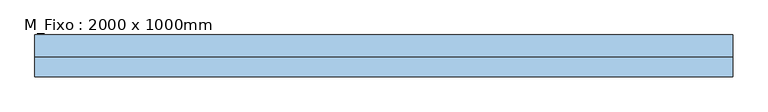
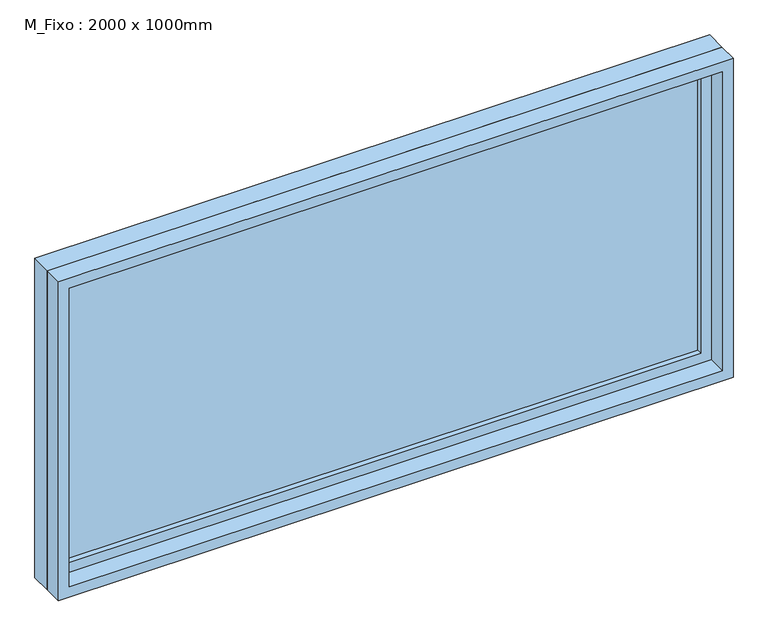
"""IFC4 building model written with IfcOpenShell, lengths in millimetres: window geometry, M_Fixo : 2000 x 1000mm."""

from ifc_helpers import new_model, si_unit, frame, origin, place, context, project, spatial, polyline, outline, extrude, source, transform, mapped, element, save


def m_fixo_2000_x_1000mm_897e8a61(model_context):
    return source(origin(), model_context, "Body", "SweptSolid", [
        extrude(outline(polyline([(-937.0, 38.0), (937.0, 38.0), (937.0, 26.0), (-937.0, 26.0), (-937.0, 38.0)])), frame((0.0, 0.0, 978.0), z_axis=(0.0, 0.0, 1.0), x_axis=(1.0, 0.0, 0.0)), (0.0, 0.0, 1.0), 874.0),
        extrude(outline(polyline([(1896.0, -981.0), (934.0, -981.0), (934.0, 981.0), (1896.0, 981.0), (1896.0, -981.0)]), holes=[polyline([(1852.0, -937.0), (1852.0, 937.0), (978.0, 937.0), (978.0, -937.0), (1852.0, -937.0)])]), frame((0.0, 10.0, 0.0), z_axis=(0.0, 1.0, 0.0), x_axis=(0.0, 0.0, 1.0)), (0.0, 0.0, 1.0), 44.0),
        extrude(outline(polyline([(1915.0, -1000.0), (915.0, -1000.0), (915.0, 1000.0), (1915.0, 1000.0), (1915.0, -1000.0)]), holes=[polyline([(1896.0, -981.0), (1896.0, 981.0), (934.0, 981.0), (934.0, -981.0), (1896.0, -981.0)])]), frame((0.0, 10.0, 0.0), z_axis=(0.0, 1.0, 0.0), x_axis=(0.0, 0.0, 1.0)), (0.0, 0.0, 1.0), 63.0),
        extrude(outline(polyline([(1915.0, -1000.0), (915.0, -1000.0), (915.0, 1000.0), (1915.0, 1000.0), (1915.0, -1000.0)]), holes=[polyline([(1883.0, -968.0), (1883.0, 968.0), (947.0, 968.0), (947.0, -968.0), (1883.0, -968.0)])]), frame((0.0, -47.0, 0.0), z_axis=(0.0, 1.0, 0.0), x_axis=(0.0, 0.0, 1.0)), (0.0, 0.0, 1.0), 57.0),
    ])


if __name__ == "__main__":
    model = new_model("IFC4")
    model_context = context("Model", 3, world=origin())
    ifc_project = project(units=[si_unit("LENGTHUNIT", "METRE", prefix="MILLI")], contexts=[model_context])
    site = spatial("IfcSite", under=ifc_project)
    building = spatial("IfcBuilding", under=site)
    placement = place(None, origin())
    m_fixo_2000_x_1000mm_shape = m_fixo_2000_x_1000mm_897e8a61(model_context)
    element("IfcWindow", 1, ObjectType="M_Fixo : 2000 x 1000mm", at=placement, inside=building, context=model_context, shape_type="MappedRepresentation", body=[
        mapped(m_fixo_2000_x_1000mm_shape, transform((0.0, 0.0, 0.0), x_axis=(1.0, 0.0, 0.0), y_axis=(0.0, 1.0, 0.0), z_axis=(0.0, 0.0, 1.0))),
    ])
    save(model, "model.ifc")

# Revit data of these elements
# Type "M_Fixo : 2000 x 1000mm"
#   Type Mark = "19"
#   Construction Type Id = "GSP4R"
#   Analytic Construction = "Vidraça única Pilkington 1/8 pol"
#   Visual Light Transmittance = 0.9
#   Thermal Resistance (R) = 0.271106 (m²·K)/W
#   Solar Heat Gain Coefficient = 0.78
#   Heat Transfer Coefficient (U) = 3.6886 W/(m²·K)
#   Height = 1.00 m
#   Altura-padrão do peitoril = 0.915 m
#   Width = 2.00 m
#   Janela aplicada = 0.019 m
#   Define Thermal Properties by = 1
#   Material da estrutura externa = Caixilho
#   Material da estrutura interna = Caixilho
#   Material do painel de vidro = Vidro
#   Caixilho = Caixilho
#   Wall Closure = (empty or 0)
# Element 1 (IfcWindow, "M_Fixo : 2000 x 1000mm")
#   Materials on its faces: "Caixilho", "Vidro"
# Materials
#   "Caixilho": class "Madeira", colour RGB 224 178 126, transparency 0, Cost = 0
#   "Vidro": class "Vidro", colour RGB 0 128 192, transparency 0.9, Description = "Vidro de sílica", Cost = 0
